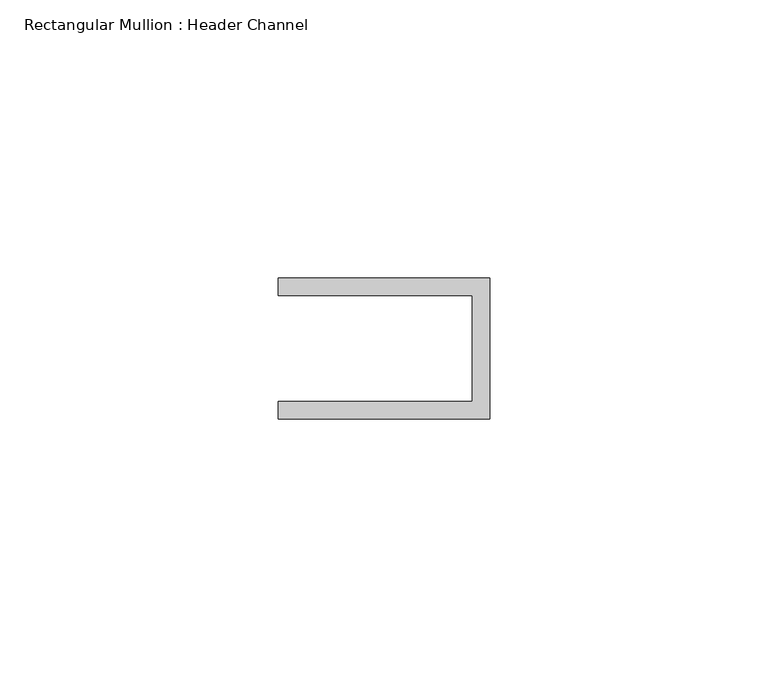
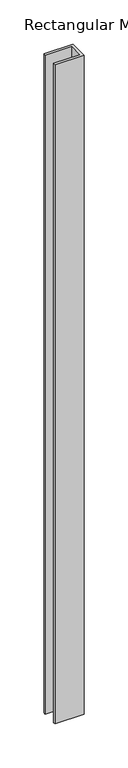
"""IFC4 building model written with IfcOpenShell, lengths in millimetres: member geometry, Rectangular Mullion : Header Channel."""

from ifc_helpers import new_model, si_unit, frame, origin, place, context, project, spatial, polyline, outline, extrude, source, transform, mapped, element, save


def rectangular_mullion_header_channel_e41eb503(model_context):
    return source(origin(), model_context, "Body", "SweptSolid", [
        extrude(outline(polyline([(0.0, 12.7), (0.0, -12.7), (-38.1, -12.7), (-38.1, -9.525), (-3.175, -9.525), (-3.175, 9.525), (-38.1, 9.525), (-38.1, 12.7), (0.0, 12.7)])), frame((0.0, 0.0, -914.4), z_axis=(0.0, 0.0, 1.0), x_axis=(1.0, 0.0, 0.0)), (0.0, 0.0, 1.0), 914.4),
    ])


if __name__ == "__main__":
    model = new_model("IFC4")
    model_context = context("Model", 3, world=origin())
    ifc_project = project(units=[si_unit("LENGTHUNIT", "METRE", prefix="MILLI")], contexts=[model_context])
    site = spatial("IfcSite", under=ifc_project)
    building = spatial("IfcBuilding", under=site)
    placement = place(None, origin())
    rectangular_mullion_header_channel_shape = rectangular_mullion_header_channel_e41eb503(model_context)
    element("IfcMember", 1, ObjectType="Rectangular Mullion : Header Channel", at=placement, inside=building, context=model_context, shape_type="MappedRepresentation", body=[
        mapped(rectangular_mullion_header_channel_shape, transform((0.0, 0.0, 0.0), x_axis=(1.0, 0.0, 0.0), y_axis=(0.0, 1.0, 0.0), z_axis=(0.0, 0.0, 1.0))),
    ])
    save(model, "model.ifc")

# Revit data of these elements
# Type "Rectangular Mullion : Header Channel"
#   built-in parameter 1007322 = 0.0833333 (stored number, unit not read)
#   built-in parameter 1007321 = -0.03125 (stored number, unit not read)
#   built-in parameter 1007320 = 0.0416667 (stored number, unit not read)
# Element 1 (IfcMember, "Rectangular Mullion : Header Channel")
#   Materials on its faces: "ALUM"
# Materials
#   "ALUM": class "Generic", colour RGB 157 157 157, transparency 0, Cost = 0
